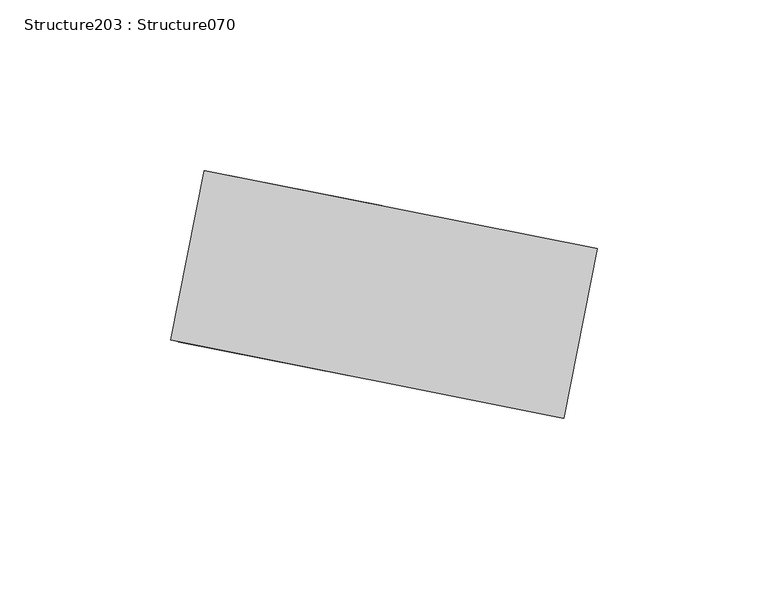
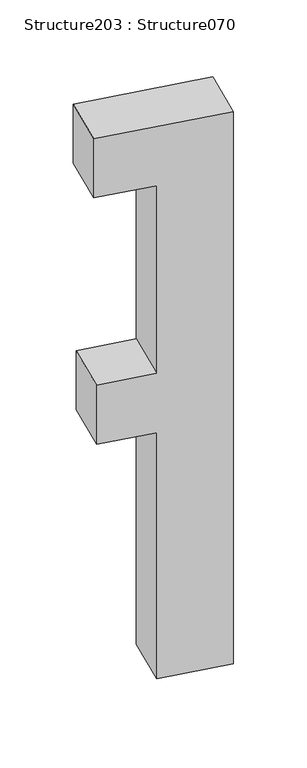
"""IFC4 building model written with IfcOpenShell, lengths in millimetres: proxy geometry, Structure203 : Structure070."""

from ifc_helpers import new_model, si_unit, frame, origin, place, context, project, spatial, polyline, outline, extrude, source, transform, mapped, element, save


def structure203_structure070_1f05042e(model_context):
    return source(origin(), model_context, "Body", "SweptSolid", [
        extrude(outline(polyline([(537.7810299, 0.0), (537.7810299, -117.5476553), (480.1634256, -117.5476553), (480.1634256, -64.5410676), (297.3185942, -64.5410676), (297.3185942, -115.249797), (239.6949411, -115.249797), (239.6949411, -64.5410676), (0.0, -64.5410676), (0.0, 0.0), (537.7810299, 0.0)])), frame((-2392.3421752, 234943.2589312, 595.2038833), z_axis=(0.19466222296394123, 0.9808703374813295, 0.0), x_axis=(0.0, 0.0, 1.0)), (0.0, 0.0, 1.0), 50.8),
    ])


if __name__ == "__main__":
    model = new_model("IFC4")
    model_context = context("Model", 3, world=origin())
    ifc_project = project(units=[si_unit("LENGTHUNIT", "METRE", prefix="MILLI")], contexts=[model_context])
    site = spatial("IfcSite", under=ifc_project)
    building = spatial("IfcBuilding", under=site)
    placement = place(None, origin())
    structure203_structure070_shape = structure203_structure070_1f05042e(model_context)
    element("IfcBuildingElementProxy", 1, Name="Structure203 : Structure070", ObjectType="Structure203 : Structure070", at=placement, inside=building, context=model_context, shape_type="MappedRepresentation", body=[
        mapped(structure203_structure070_shape, transform((0.0, 0.0, 0.0), x_axis=(1.0, 0.0, 0.0), y_axis=(0.0, 1.0, 0.0), z_axis=(0.0, 0.0, 1.0))),
    ])
    save(model, "model.ifc")

# Revit data of these elements
# Type "Structure203 : Structure070"
#   NameOverride = "Structure070"
# Element 1 (IfcBuildingElementProxy, "Structure203 : Structure070")
#   Materials on its faces: "BRUSHED ALUMINUM LETTERING"
# Materials
#   "BRUSHED ALUMINUM LETTERING": class "Unassigned", colour RGB 169 181 186, transparency 0, Cost = 0
